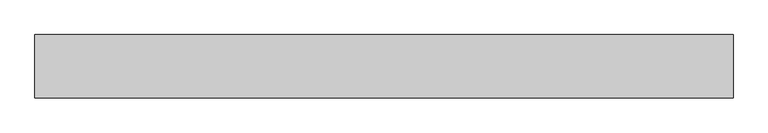
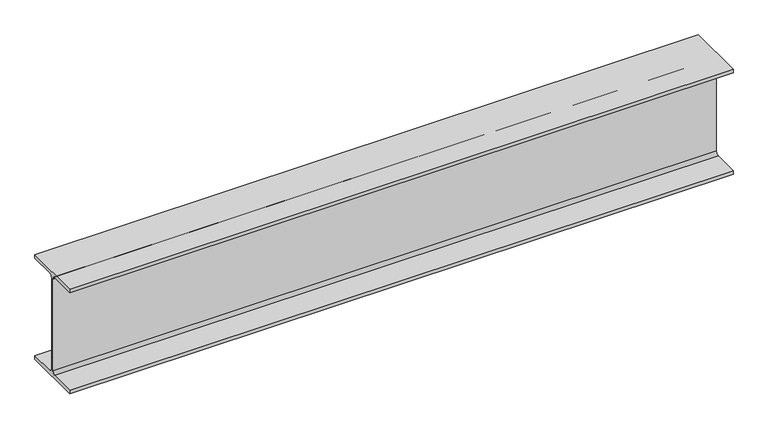
"""IFC4 building model written with IfcOpenShell, lengths in millimetres: beam geometry, Steel Beam_H-KSD3502 : H_SB_ASB_H-200x200x8x12."""

from ifc_helpers import new_model, si_unit, point, frame, frame_2d, origin, place, context, project, spatial, polyline, circle_curve, trimmed, segment, composite_curve, outline, extrude, source, transform, mapped, element, save


def beam_2b48dec8(model_context):
    return source(origin(), model_context, "Body", "SweptSolid", [
        extrude(outline(composite_curve([segment(polyline([(82.5, -141.5), (82.5, -151.7), (-82.5, -151.7), (-82.5, -141.5), (-11.9, -141.5)]), True, "CONTINUOUS"), segment(trimmed(circle_curve(frame_2d((-11.9, -132.6)), 8.9), [point((-11.9, -141.5))], [point((-3.0, -132.6))], True, "CARTESIAN"), True, "CONTINUOUS"), segment(polyline([(-3.0, -132.6), (-3.0, 132.6)]), True, "CONTINUOUS"), segment(trimmed(circle_curve(frame_2d((-11.9, 132.6)), 8.9), [point((-3.0, 132.6))], [point((-11.9, 141.5))], True, "CARTESIAN"), True, "CONTINUOUS"), segment(polyline([(-11.9, 141.5), (-82.5, 141.5), (-82.5, 151.7), (82.5, 151.7), (82.5, 141.5), (11.9, 141.5)]), True, "CONTINUOUS"), segment(trimmed(circle_curve(frame_2d((11.9, 132.6)), 8.9), [point((11.9, 141.5))], [point((3.0, 132.6))], True, "CARTESIAN"), True, "CONTINUOUS"), segment(polyline([(3.0, 132.6), (3.0, -132.6)]), True, "CONTINUOUS"), segment(trimmed(circle_curve(frame_2d((11.9, -132.6)), 8.9), [point((3.0, -132.6))], [point((11.9, -141.5))], True, "CARTESIAN"), True, "CONTINUOUS"), segment(polyline([(11.9, -141.5), (82.5, -141.5)]), True, "CONTINUOUS")], self_intersect=False)), frame((-1035.0333333, 0.0, 0.0), z_axis=(1.0, 0.0, 0.0), x_axis=(0.0, 1.0, 0.0)), (0.0, 0.0, 1.0), 1820.0666667),
    ])


if __name__ == "__main__":
    model = new_model("IFC4")
    model_context = context("Model", 3, world=origin())
    ifc_project = project(units=[si_unit("LENGTHUNIT", "METRE", prefix="MILLI")], contexts=[model_context])
    site = spatial("IfcSite", under=ifc_project)
    building = spatial("IfcBuilding", under=site)
    placement = place(None, origin())
    beam_shape = beam_2b48dec8(model_context)
    element("IfcBeam", 1, ObjectType="Steel Beam_H-KSD3502 : H_SB_ASB_H-200x200x8x12", at=placement, inside=building, context=model_context, shape_type="MappedRepresentation", body=[
        mapped(beam_shape, transform((0.0, 0.0, 0.0), x_axis=(1.0, 0.0, 0.0), y_axis=(0.0, 1.0, 0.0), z_axis=(0.0, 0.0, 1.0))),
    ])
    save(model, "model.ifc")

# Revit data of these elements
# Type "Steel Beam_H-KSD3502 : H_SB_ASB_H-200x200x8x12"
#   Width = 20.0 cm
#   Web Thickness = 0.8 cm
#   Web Fillet = 1.3 cm
#   Warping Constant = 141376.0 cm⁶
#   Torsional Moment of Inertia = 26.2485 cm⁴
#   Torsional Modulus = 1.0 cm³
#   Section Area = 63.53 cm²
#   Plastic Modulus weak axis = 244.0 cm³
#   Plastic Modulus strong axis = 525.0 cm³
#   Perimeter = 1.16 m²/m
#   Nominal Weight = 49.90 kgf/m
#   Moment of Inertia weak axis = 1600.00 cm⁴
#   Moment of Inertia strong axis = 4720.00 cm⁴
#   Height = 20.0 cm
#   Flange Thickness = 1.2 cm
#   Elastic Modulus weak axis = 160.0 cm³
#   Elastic Modulus strong axis = 472.0 cm³
#   Centroid Vertical = 10.0 cm
#   Centroid Horizontal = 10.0 cm
#   Length [instance default] = 1.5240 m
#   Structural Material [instance default] = Steel, 45-345
#   Assembly Code = ""
# Element 1 (IfcBeam, "Steel Beam_H-KSD3502 : H_SB_ASB_H-200x200x8x12")
#   Structural Material = none
# Materials
#   "Steel, 45-345": class "Metal", colour RGB 189 187 185, transparency 0, Description = "Steel 345 MPa", Cost = 0
